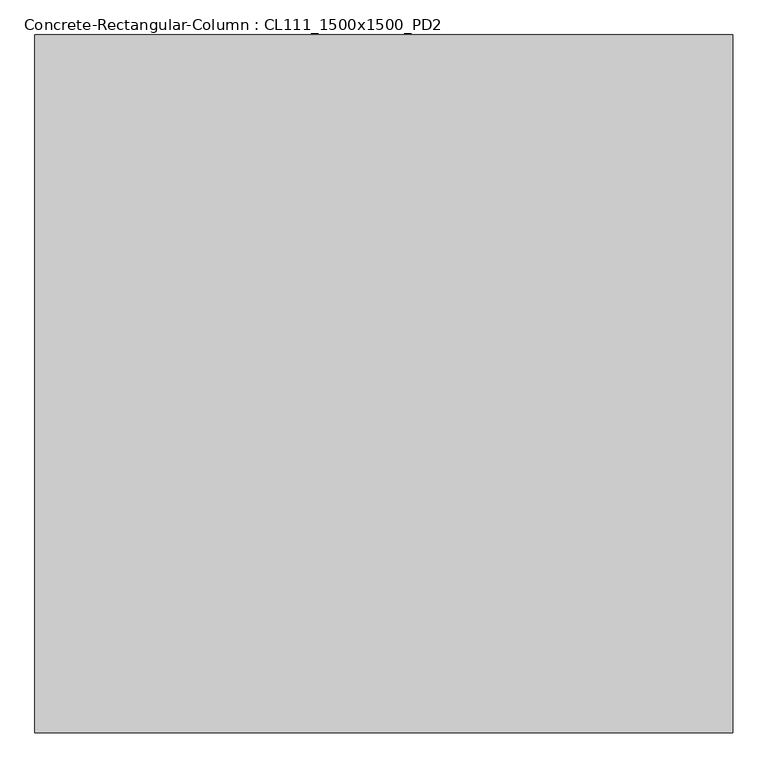
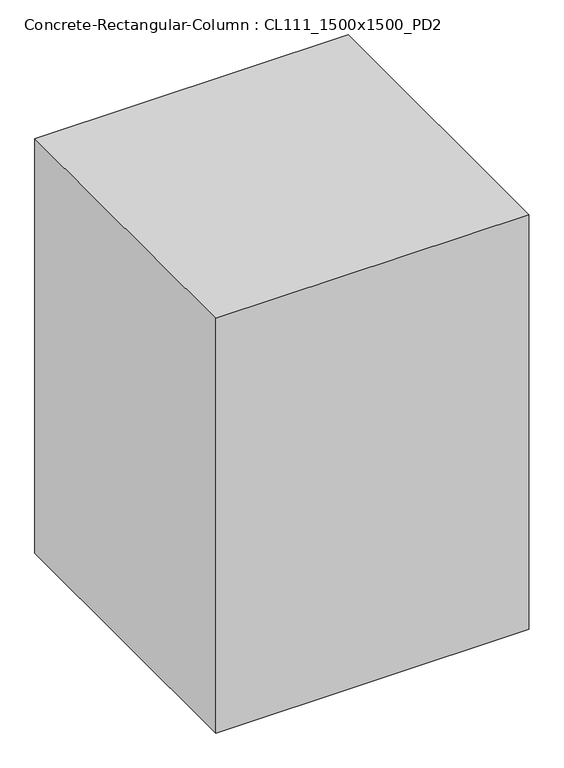
"""IFC4 building model written with IfcOpenShell, lengths in millimetres: column geometry, Concrete-Rectangular-Column : CL111_1500x1500_PD2."""

from ifc_helpers import new_model, si_unit, frame, origin, place, context, project, spatial, polyline, outline, extrude, source, transform, mapped, element, save


def concrete_rectangular_column_cl111_1500x1500_pd2_705c837b(model_context):
    return source(origin(), model_context, "Body", "SweptSolid", [
        extrude(outline(polyline([(750.0, 750.0), (750.0, -750.0), (-750.0, -750.0), (-750.0, 750.0), (750.0, 750.0)])), frame((0.0, 0.0, -2100.0), z_axis=(0.0, 0.0, 1.0), x_axis=(1.0, 0.0, 0.0)), (0.0, 0.0, 1.0), 2100.0),
    ])


if __name__ == "__main__":
    model = new_model("IFC4")
    model_context = context("Model", 3, world=origin())
    ifc_project = project(units=[si_unit("LENGTHUNIT", "METRE", prefix="MILLI")], contexts=[model_context])
    site = spatial("IfcSite", under=ifc_project)
    building = spatial("IfcBuilding", under=site)
    placement = place(None, origin())
    concrete_rectangular_column_cl111_1500x1500_pd2_shape = concrete_rectangular_column_cl111_1500x1500_pd2_705c837b(model_context)
    element("IfcColumn", 1, ObjectType="Concrete-Rectangular-Column : CL111_1500x1500_PD2", at=placement, inside=building, context=model_context, shape_type="MappedRepresentation", body=[
        mapped(concrete_rectangular_column_cl111_1500x1500_pd2_shape, transform((0.0, 0.0, 0.0), x_axis=(1.0, 0.0, 0.0), y_axis=(0.0, 1.0, 0.0), z_axis=(0.0, 0.0, 1.0))),
    ])
    save(model, "model.ifc")

# Revit data of these elements
# Type "Concrete-Rectangular-Column : CL111_1500x1500_PD2"
#   Description = "UG 철골 기둥용 Pedestal"
#   b = 1500 mm
#   h = 1500 mm
#   Width = 1500 mm
#   Length = 1500 mm
#   hec_material3 [instance default] = none
#   hec_material2 [instance default] = A03AE056-00001_Bitumen/Bituminous/Asphalt Coating
#   hec_material1 [instance default] = A03AC035-00001_Form Work (3 times in use)_Flat
#   Structural Material [instance default] = A03AC032-00007_Structural Concrete_Type1_25MPa-30Mpa
# Element 1 (IfcColumn, "Concrete-Rectangular-Column : CL111_1500x1500_PD2")
#   hec_material2 = none
#   hec_material1 = none
#   Structural Material = 콘크리트 - 현장타설 콘크리트
#   Materials on its faces: "콘크리트 - 현장타설 콘크리트"
# Materials
#   "A03AE056-00001_Bitumen/Bituminous/Asphalt Coating": class "Generic", colour RGB 17 17 17, transparency 0, Description = "Damp-proofing", W00) Work Master Code = "A03AE056-00001", W01) Work Master_Lv1 = "Concrete Work", W02) Work Master_Lv2 = "Concrete Protective Coating (U/G)", W03) Work Master_Spec.1 = "Bitumen/Bituminous/Asphalt Coating", Cost = 0
#   "A03AC035-00001_Form Work (3 times in use)_Flat": class "Wood", colour RGB 149 120 74, transparency 0, Description = "Plywood", W00) Work Master Code = "A03AC035-00001", W01) Work Master_Lv1 = "Concrete Work", W02) Work Master_Lv2 = "Substructure Work", W03) Work Master_Spec.1 = "Form Work (3 times in use)", W04) Work Master_Spec.2 = "Flat Form", W05) Work Master_Spec.3 = "Dressed Lumber, Plywood or Steel Form(Wood Planks are not Allowed) incl. Chamfer", Cost = 0
#   "A03AC032-00007_Structural Concrete_Type1_25MPa-30Mpa": class "Concrete", colour RGB 176 176 176, transparency 0, Keynote = "09910.A1", Description = "Reinf. Conc.", W00) Work Master Code = "A03AC032-00007", W01) Work Master_Lv1 = "Concrete Work", W02) Work Master_Lv2 = "Substructure Work", W03) Work Master_Spec.1 = "Structural Concrete", W04) Work Master_Spec.2 = "Cement Type-1", W05) Work Master_Spec.3 = "25MPa < F'c (Cylinder Strength) ≤ 30MPa", Cost = 0
#   "콘크리트 - 현장타설 콘크리트": class "콘크리트", colour RGB 192 192 192, transparency 0
